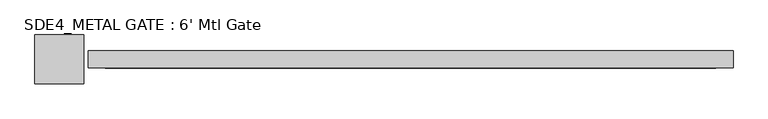
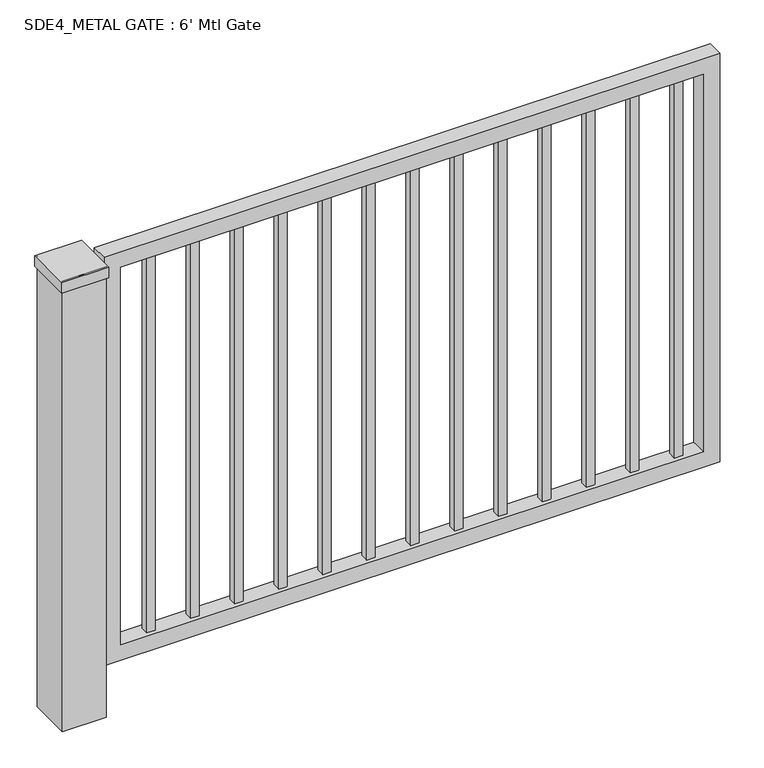
"""IFC4 building model written with IfcOpenShell, lengths in millimetres: proxy geometry, SDE4_METAL GATE : 6' Mtl Gate."""

from ifc_helpers import new_model, si_unit, frame, origin, origin_with_axes, place, context, project, spatial, polyline, outline, extrude, source, transform, mapped, element, save


def sde4_metal_gate_6_mtl_gate_23c9f4d1(model_context):
    return source(origin(), model_context, "Body", "SweptSolid", [
        extrude(outline(polyline([(1406.525, 9.525), (1406.525, -9.525), (1387.475, -9.525), (1387.475, 9.525), (1406.525, 9.525)])), frame((0.0, 0.0, 139.7), z_axis=(0.0, 0.0, 1.0), x_axis=(1.0, 0.0, 0.0)), (0.0, 0.0, 1.0), 950.0),
        extrude(outline(polyline([(1304.925, 9.525), (1304.925, -9.525), (1285.875, -9.525), (1285.875, 9.525), (1304.925, 9.525)])), frame((0.0, 0.0, 139.7), z_axis=(0.0, 0.0, 1.0), x_axis=(1.0, 0.0, 0.0)), (0.0, 0.0, 1.0), 950.0),
        extrude(outline(polyline([(1203.325, 9.525), (1203.325, -9.525), (1184.275, -9.525), (1184.275, 9.525), (1203.325, 9.525)])), frame((0.0, 0.0, 139.7), z_axis=(0.0, 0.0, 1.0), x_axis=(1.0, 0.0, 0.0)), (0.0, 0.0, 1.0), 950.0),
        extrude(outline(polyline([(1101.725, 9.525), (1101.725, -9.525), (1082.675, -9.525), (1082.675, 9.525), (1101.725, 9.525)])), frame((0.0, 0.0, 139.7), z_axis=(0.0, 0.0, 1.0), x_axis=(1.0, 0.0, 0.0)), (0.0, 0.0, 1.0), 950.0),
        extrude(outline(polyline([(1000.125, 9.525), (1000.125, -9.525), (981.075, -9.525), (981.075, 9.525), (1000.125, 9.525)])), frame((0.0, 0.0, 139.7), z_axis=(0.0, 0.0, 1.0), x_axis=(1.0, 0.0, 0.0)), (0.0, 0.0, 1.0), 950.0),
        extrude(outline(polyline([(898.525, 9.525), (898.525, -9.525), (879.475, -9.525), (879.475, 9.525), (898.525, 9.525)])), frame((0.0, 0.0, 139.7), z_axis=(0.0, 0.0, 1.0), x_axis=(1.0, 0.0, 0.0)), (0.0, 0.0, 1.0), 950.0),
        extrude(outline(polyline([(796.925, 9.525), (796.925, -9.525), (777.875, -9.525), (777.875, 9.525), (796.925, 9.525)])), frame((0.0, 0.0, 139.7), z_axis=(0.0, 0.0, 1.0), x_axis=(1.0, 0.0, 0.0)), (0.0, 0.0, 1.0), 950.0),
        extrude(outline(polyline([(695.325, 9.525), (695.325, -9.525), (676.275, -9.525), (676.275, 9.525), (695.325, 9.525)])), frame((0.0, 0.0, 139.7), z_axis=(0.0, 0.0, 1.0), x_axis=(1.0, 0.0, 0.0)), (0.0, 0.0, 1.0), 950.0),
        extrude(outline(polyline([(593.725, 9.525), (593.725, -9.525), (574.675, -9.525), (574.675, 9.525), (593.725, 9.525)])), frame((0.0, 0.0, 139.7), z_axis=(0.0, 0.0, 1.0), x_axis=(1.0, 0.0, 0.0)), (0.0, 0.0, 1.0), 950.0),
        extrude(outline(polyline([(492.125, 9.525), (492.125, -9.525), (473.075, -9.525), (473.075, 9.525), (492.125, 9.525)])), frame((0.0, 0.0, 139.7), z_axis=(0.0, 0.0, 1.0), x_axis=(1.0, 0.0, 0.0)), (0.0, 0.0, 1.0), 950.0),
        extrude(outline(polyline([(390.525, 9.525), (390.525, -9.525), (371.475, -9.525), (371.475, 9.525), (390.525, 9.525)])), frame((0.0, 0.0, 139.7), z_axis=(0.0, 0.0, 1.0), x_axis=(1.0, 0.0, 0.0)), (0.0, 0.0, 1.0), 950.0),
        extrude(outline(polyline([(288.925, 9.525), (288.925, -9.525), (269.875, -9.525), (269.875, 9.525), (288.925, 9.525)])), frame((0.0, 0.0, 139.7), z_axis=(0.0, 0.0, 1.0), x_axis=(1.0, 0.0, 0.0)), (0.0, 0.0, 1.0), 950.0),
        extrude(outline(polyline([(187.325, 9.525), (187.325, -9.525), (168.275, -9.525), (168.275, 9.525), (187.325, 9.525)])), frame((0.0, 0.0, 139.7), z_axis=(0.0, 0.0, 1.0), x_axis=(1.0, 0.0, 0.0)), (0.0, 0.0, 1.0), 950.0),
        extrude(outline(polyline([(53.975, -53.975), (-53.975, -53.975), (-53.975, 53.975), (53.975, 53.975), (53.975, -53.975)])), frame((0.0, 0.0, 1074.6), z_axis=(0.0, 0.0, 1.0), x_axis=(1.0, 0.0, 0.0)), (0.0, 0.0, 1.0), 25.4),
        extrude(outline(polyline([(50.8, 50.8), (50.8, -50.8), (-50.8, -50.8), (-50.8, 50.8), (50.8, 50.8)])), origin_with_axes(), (0.0, 0.0, 1.0), 1100.0),
        extrude(outline(polyline([(101.6, 1487.3), (1100.0, 1487.3), (1100.0, 63.5), (101.6, 63.5), (101.6, 1487.3)]), holes=[polyline([(1061.9, 1449.2), (139.7, 1449.2), (139.7, 101.6), (1061.9, 101.6), (1061.9, 1449.2)])]), frame((0.0, -19.05, 0.0), z_axis=(0.0, 1.0, 0.0), x_axis=(0.0, 0.0, 1.0)), (0.0, 0.0, 1.0), 38.1),
    ])


if __name__ == "__main__":
    model = new_model("IFC4")
    model_context = context("Model", 3, world=origin())
    ifc_project = project(units=[si_unit("LENGTHUNIT", "METRE", prefix="MILLI")], contexts=[model_context])
    site = spatial("IfcSite", under=ifc_project)
    building = spatial("IfcBuilding", under=site)
    placement = place(None, origin())
    sde4_metal_gate_6_mtl_gate_shape = sde4_metal_gate_6_mtl_gate_23c9f4d1(model_context)
    element("IfcBuildingElementProxy", 1, Name="SDE4_METAL GATE : 6' Mtl Gate", ObjectType="SDE4_METAL GATE : 6' Mtl Gate", at=placement, inside=building, context=model_context, shape_type="MappedRepresentation", body=[
        mapped(sde4_metal_gate_6_mtl_gate_shape, transform((0.0, 0.0, 0.0), x_axis=(1.0, 0.0, 0.0), y_axis=(0.0, 1.0, 0.0), z_axis=(0.0, 0.0, 1.0))),
    ])
    save(model, "model.ifc")

# Revit data of these elements
# Type "SDE4_METAL GATE : 6' Mtl Gate"
#   Type Mark = "G3"
#   Keynote = "2.26"
#   Swing Angle [instance default] = 90.00°
#   Post Height [instance default] = 1905.00 mm
#   Picket Heght [instance default] = 1651.00 mm
#   Width [instance default] = 1219.20 mm
#   Gate Height [instance default] = 1828.80 mm
#   Upper Picket Array [instance default] = 5
#   Lower Picket Array [instance default] = 10
#   Assembly Code = ""
# Element 1 (IfcBuildingElementProxy, "SDE4_METAL GATE : 6' Mtl Gate")
#   Post Height = 1176.20 mm
#   Picket Heght = 950.00 mm
#   Width = 1500.00 mm
#   Gate Height = 1100.00 mm
#   Upper Picket Array = 6
#   Lower Picket Array = 13
